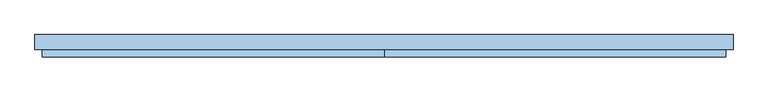
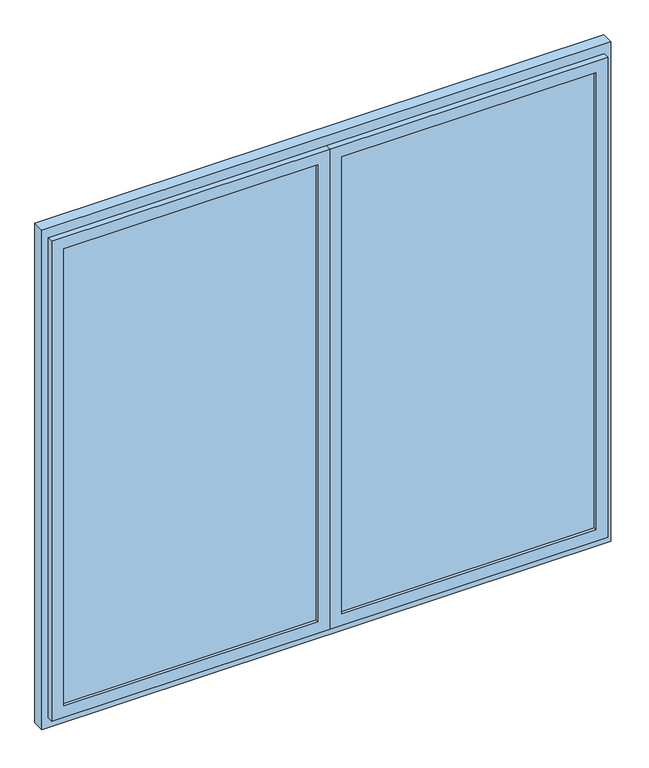
"""IFC4 building model written with IfcOpenShell, lengths in millimetres: window geometry, Fenstertür 2-flg : Fenstertür 2-flg 2.8x2.6."""

from ifc_helpers import new_model, si_unit, frame, origin, place, context, project, spatial, polyline, outline, extrude, faceted_brep, source, transform, mapped, element, save


def window_6f00e414(model_context):
    return source(origin(), model_context, "Body", "SolidModel", [
        extrude(outline(polyline([(30.0, -15.0), (-30.0, -15.0), (-30.0, 45.0), (30.0, 45.0), (30.0, -15.0)])), frame((0.0, 0.0, 80.0), z_axis=(0.0, 0.0, 1.0), x_axis=(1.0, 0.0, 0.0)), (0.0, 0.0, 1.0), 2440.0),
        extrude(outline(polyline([(2600.0, -1400.0), (0.0, -1400.0), (0.0, 1400.0), (2600.0, 1400.0), (2600.0, -1400.0)]), holes=[polyline([(2520.0, -1340.0), (2520.0, 1340.0), (80.0, 1340.0), (80.0, -1340.0), (2520.0, -1340.0)])]), frame((0.0, -15.0, 0.0), z_axis=(0.0, 1.0, 0.0), x_axis=(0.0, 0.0, 1.0)), (0.0, 0.0, 1.0), 60.0),
        faceted_brep([(-1340.0, -15.0, 80.0), (-1340.0, 15.0, 80.0), (-30.0, 15.0, 80.0), (-30.0, -15.0, 80.0), (-30.0, 15.0, 2520.0), (-30.0, -15.0, 2520.0), (-1340.0, 15.0, 2520.0), (-60.0, 15.0, 2490.0), (-1310.0, 15.0, 2490.0), (-1310.0, 15.0, 110.0), (-60.0, 15.0, 110.0), (0.0, -15.0, 50.0), (-1370.0, -15.0, 50.0), (-1370.0, -15.0, 2550.0), (0.0, -15.0, 2550.0), (-1340.0, -15.0, 2520.0), (-1370.0, -45.0, 50.0), (0.0, -45.0, 50.0), (0.0, -45.0, 2550.0), (-1370.0, -45.0, 2550.0), (-60.0, -45.0, 110.0), (-1310.0, -45.0, 110.0), (-1310.0, -45.0, 2490.0), (-60.0, -45.0, 2490.0)], [[[0, 1, 2, 3]], [[3, 2, 4, 5]], [[2, 1, 6, 4], [7, 8, 9, 10]], [[11, 12, 13, 14], [5, 15, 0, 3]], [[16, 12, 11, 17]], [[17, 11, 14, 18]], [[18, 19, 16, 17], [20, 21, 22, 23]], [[9, 21, 20, 10]], [[10, 20, 23, 7]], [[15, 6, 1, 0]], [[19, 13, 12, 16]], [[8, 22, 21, 9]], [[5, 4, 6, 15]], [[18, 14, 13, 19]], [[7, 23, 22, 8]]]),
        faceted_brep([(30.0, -15.0, 80.0), (30.0, 15.0, 80.0), (1340.0, 15.0, 80.0), (1340.0, -15.0, 80.0), (1340.0, 15.0, 2520.0), (1340.0, -15.0, 2520.0), (30.0, 15.0, 2520.0), (1310.0, 15.0, 2490.0), (60.0, 15.0, 2490.0), (60.0, 15.0, 110.0), (1310.0, 15.0, 110.0), (1370.0, -15.0, 50.0), (0.0, -15.0, 50.0), (0.0, -15.0, 2550.0), (1370.0, -15.0, 2550.0), (30.0, -15.0, 2520.0), (0.0, -45.0, 50.0), (1370.0, -45.0, 50.0), (1370.0, -45.0, 2550.0), (0.0, -45.0, 2550.0), (1310.0, -45.0, 110.0), (60.0, -45.0, 110.0), (60.0, -45.0, 2490.0), (1310.0, -45.0, 2490.0)], [[[0, 1, 2, 3]], [[3, 2, 4, 5]], [[2, 1, 6, 4], [7, 8, 9, 10]], [[11, 12, 13, 14], [5, 15, 0, 3]], [[16, 12, 11, 17]], [[17, 11, 14, 18]], [[18, 19, 16, 17], [20, 21, 22, 23]], [[9, 21, 20, 10]], [[10, 20, 23, 7]], [[15, 6, 1, 0]], [[19, 13, 12, 16]], [[8, 22, 21, 9]], [[5, 4, 6, 15]], [[18, 14, 13, 19]], [[7, 23, 22, 8]]]),
        extrude(outline(polyline([(60.0, 0.0), (1310.0, 0.0), (1310.0, -30.0), (60.0, -30.0), (60.0, 0.0)])), frame((0.0, 0.0, 110.0), z_axis=(0.0, 0.0, 1.0), x_axis=(1.0, 0.0, 0.0)), (0.0, 0.0, 1.0), 2380.0),
        extrude(outline(polyline([(-1310.0, 0.0), (-60.0, 0.0), (-60.0, -30.0), (-1310.0, -30.0), (-1310.0, 0.0)])), frame((0.0, 0.0, 110.0), z_axis=(0.0, 0.0, 1.0), x_axis=(1.0, 0.0, 0.0)), (0.0, 0.0, 1.0), 2380.0),
    ])


if __name__ == "__main__":
    model = new_model("IFC4")
    model_context = context("Model", 3, world=origin())
    ifc_project = project(units=[si_unit("LENGTHUNIT", "METRE", prefix="MILLI")], contexts=[model_context])
    site = spatial("IfcSite", under=ifc_project)
    building = spatial("IfcBuilding", under=site)
    placement = place(None, origin())
    window_shape = window_6f00e414(model_context)
    element("IfcWindow", 1, ObjectType="Fenstertür 2-flg : Fenstertür 2-flg 2.8x2.6", at=placement, inside=building, context=model_context, shape_type="MappedRepresentation", body=[
        mapped(window_shape, transform((0.0, 0.0, 0.0), x_axis=(1.0, 0.0, 0.0), y_axis=(0.0, 1.0, 0.0), z_axis=(0.0, 0.0, 1.0))),
    ])
    save(model, "model.ifc")

# Revit data of these elements
# Type "Fenstertür 2-flg : Fenstertür 2-flg 2.8x2.6"
#   Type Mark = "76"
#   Operation = "DoublePanelVertical"
#   Construction Type Id = "GSP4R"
#   Keynote = "16.05.01"
#   Analytic Construction = "1/8 Zoll Pilkington-Verglasung einfach"
#   Thermal Resistance (R) = 0.271106 (m²·K)/W
#   Visual Light Transmittance = 0.9
#   Solar Heat Gain Coefficient = 0.78
#   Rough Width = 2.800 m
#   Rough Height = 2.600 m
#   Heat Transfer Coefficient (U) = 3.6886 W/(m²·K)
#   Rahmentiefe = 0.060 m
#   Rahmenhöhe unten = 0.080 m
#   Höhe oberer  Rahmen = 0.080 m
#   Rahmenbreite = 0.060 m
#   Height = 2.600 m
#   Tiefe Flügel = 0.060 m
#   Flügelbreite = 0.060 m
#   Einbautiefe (von außen) [instance default] = 0.140 m
#   Width = 2.800 m
#   Sichtbarkeit Sturzlinien [instance default] = yes
#   Öffnungsrichtung oben [instance default] = yes
#   Öffnungsrichtung in Draufsicht anzeigen [instance default] = yes
#   Drehflügel 1 [instance default] = yes
#   Bild [instance default] = none
#   Glas [instance default] = none
#   Fensterflügel [instance default] = none
#   Äußere Fensterbank [instance default] = none
#   Innere Fensterbank [instance default] = none
#   Wall Closure = (empty or 0)
# Element 1 (IfcWindow, "Fenstertür 2-flg : Fenstertür 2-flg 2.8x2.6")
#   Einbautiefe (von außen) = 0.230 m
#   Materials on its faces: "Kunststoff - Weiß", "Glas"
# Materials
#   "Kunststoff - Weiß": class "Kunststoff", colour RGB 249 249 249, transparency 0, Cost = 0
#   "Glas": class "Glas", colour RGB 0 0 255, transparency 0.75, Comments = "Render-Darstellung nicht aktualisiert ", Cost = 0
